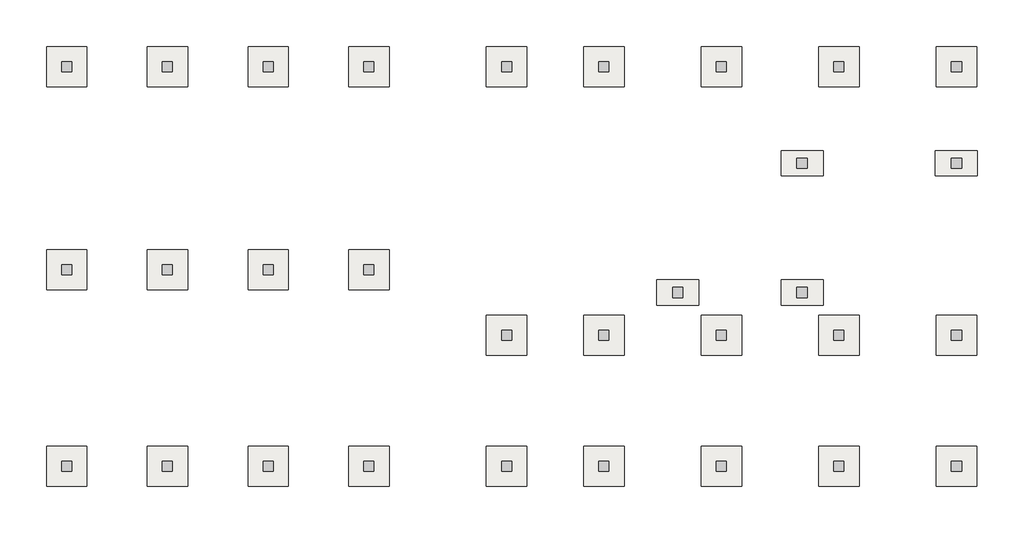
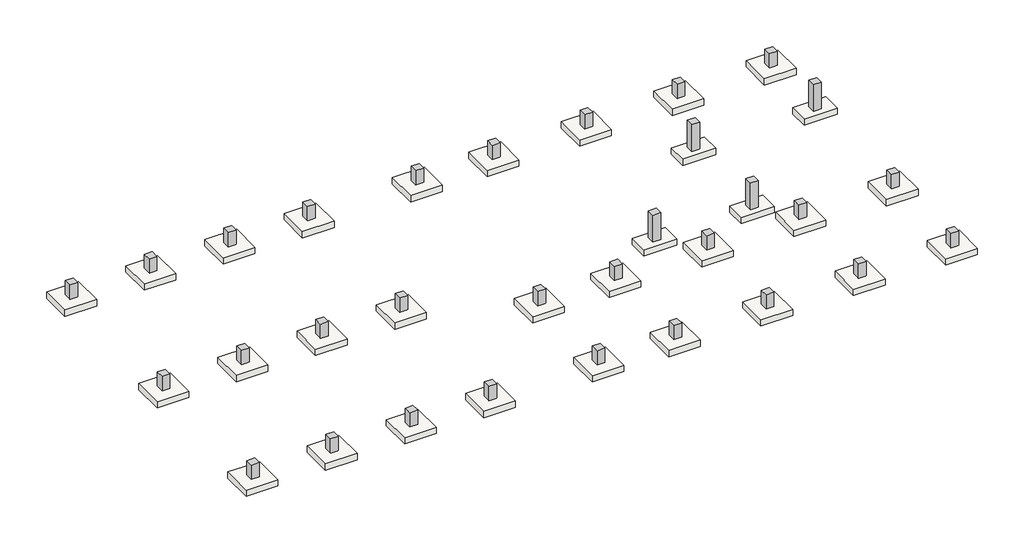
# Not in any storey: 31 columns, 31 slabs.
"""IFC4 building model written with IfcOpenShell, lengths in millimetres."""

import ifcopenshell
import ifcopenshell.guid

model = None  # the IFC model being written
_history = None  # IfcOwnerHistory: only IFC2X3 demands one
_inside = {}  # id of a spatial element -> (the spatial element, [elements in it])
_under = {}  # id of a project, library or spatial element -> (it, [spatial elements below it])
_declared = {}  # id of a project -> (the project, [libraries it declares])
_typed = {}  # id of a type object -> (the type object, [elements of that type])
_made_of = {}  # id of a material, layer set ... -> (it, [elements and type objects made of it])


def new_model(schema):
    """Start an empty IFC model of exactly this schema.

    Asked for "IFC4X3", IfcOpenShell would pick the latest addendum, in which some entities
    have other attributes; the version numbers below select the first issue.
    IFC2X3 requires an IfcOwnerHistory on every rooted entity: one is made here for all.
    """
    global model, _history
    if schema == "IFC4X3":
        model = ifcopenshell.file(schema_version=(4, 3, 0, 0))
    else:
        model = ifcopenshell.file(schema=schema)
    _inside.clear()
    _under.clear()
    _declared.clear()
    _typed.clear()
    _made_of.clear()
    _history = None
    if model.schema == "IFC2X3":
        org = make("IfcOrganization", Name="unknown")
        user = make(
            "IfcPersonAndOrganization",
            ThePerson=make("IfcPerson", FamilyName="unknown"),
            TheOrganization=org,
        )
        app = make(
            "IfcApplication",
            ApplicationDeveloper=org,
            Version="unknown",
            ApplicationFullName="unknown",
            ApplicationIdentifier="unknown",
        )
        _history = make(
            "IfcOwnerHistory",
            OwningUser=user,
            OwningApplication=app,
            ChangeAction="ADDED",
            CreationDate=0,
        )
    return model


def make(cls, **values):
    """One entity of the class cls with the attributes given. An attribute that is None is left unset."""
    return model.create_entity(
        cls, **{name: value for name, value in values.items() if value is not None}
    )


def rooted(cls, **values):
    """An entity with a GlobalId (a new one), such as an element, a storey or a relation."""
    return make(cls, GlobalId=ifcopenshell.guid.new(), OwnerHistory=_history, **values)


def si_unit(unit_type, name, prefix=None):
    """IfcSIUnit, for example si_unit("LENGTHUNIT", "METRE", prefix="MILLI")."""
    return make("IfcSIUnit", UnitType=unit_type, Prefix=prefix, Name=name)


def assignment(units):
    """IfcUnitAssignment: the units of a project."""
    return None if units is None else make("IfcUnitAssignment", Units=units)


def point(xyz):
    """IfcCartesianPoint."""
    return None if xyz is None else make("IfcCartesianPoint", Coordinates=xyz)


def direction(xyz):
    """IfcDirection."""
    return None if xyz is None else make("IfcDirection", DirectionRatios=xyz)


def frame(location, z_axis=None, x_axis=None):
    """IfcAxis2Placement3D, a coordinate frame: its origin and axes. An axis left out is left unset."""
    return make(
        "IfcAxis2Placement3D",
        Location=point(location),
        Axis=direction(z_axis),
        RefDirection=direction(x_axis),
    )


def origin():
    """The frame at (0, 0, 0) with its axes left unset."""
    return frame((0.0, 0.0, 0.0))


def place(relative_to, where):
    """IfcLocalPlacement: puts the frame where relative to a parent placement (None: the world)."""
    return make(
        "IfcLocalPlacement", PlacementRelTo=relative_to, RelativePlacement=where
    )


def context(
    kind, dimensions, precision=None, world=None, true_north=None, identifier=None
):
    """IfcGeometricRepresentationContext, for example the 3D "Model" context."""
    return make(
        "IfcGeometricRepresentationContext",
        ContextIdentifier=identifier,
        ContextType=kind,
        CoordinateSpaceDimension=dimensions,
        Precision=precision,
        WorldCoordinateSystem=world,
        TrueNorth=true_north,
    )


def project(units=None, contexts=None):
    """IfcProject with its units and contexts."""
    return rooted(
        "IfcProject",
        Name="project",
        RepresentationContexts=contexts,
        UnitsInContext=assignment(units),
    )


def spatial(cls, under=None, at=None, **own):
    """A site, building, storey or space (cls), placed at a placement, below another one or the project."""
    s = rooted(cls, ObjectPlacement=at, **own)
    if under is not None:
        _under.setdefault(under.id(), (under, []))[1].append(s)
    return s


def polyline(points):
    """IfcPolyline through the points."""
    return make("IfcPolyline", Points=[point(p) for p in points])


def outline(outer, holes=None, kind="AREA"):
    """IfcArbitraryClosedProfileDef: a profile drawn as a closed curve; with holes, ...WithVoids."""
    if holes is None:
        return make("IfcArbitraryClosedProfileDef", ProfileType=kind, OuterCurve=outer)
    return make(
        "IfcArbitraryProfileDefWithVoids",
        ProfileType=kind,
        OuterCurve=outer,
        InnerCurves=holes,
    )


def extrude(swept, where, along, depth):
    """IfcExtrudedAreaSolid: the profile swept, set in the frame where, extruded along a direction by depth."""
    return make(
        "IfcExtrudedAreaSolid",
        SweptArea=swept,
        Position=where,
        ExtrudedDirection=direction(along),
        Depth=depth,
    )


def shape(context_of_items, identifier, shape_type, items):
    """IfcShapeRepresentation: the items that make up one representation, for example the "Body"."""
    return make(
        "IfcShapeRepresentation",
        ContextOfItems=context_of_items,
        RepresentationIdentifier=identifier,
        RepresentationType=shape_type,
        Items=items,
    )


def source(mapping_origin, context_of_items, identifier, shape_type, items):
    """IfcRepresentationMap: a shape defined once, which mapped items show again and again."""
    return make(
        "IfcRepresentationMap",
        MappingOrigin=mapping_origin,
        MappedRepresentation=shape(context_of_items, identifier, shape_type, items),
    )


def transform(
    local_origin,
    x_axis=None,
    y_axis=None,
    z_axis=None,
    scale=None,
    scale2=None,
    scale3=None,
    uniform=True,
):
    """IfcCartesianTransformationOperator3D, or its non-uniform kind. x_axis, y_axis, z_axis: its Axis1, 2, 3."""
    if uniform:
        return make(
            "IfcCartesianTransformationOperator3D",
            Axis1=direction(x_axis),
            Axis2=direction(y_axis),
            LocalOrigin=point(local_origin),
            Scale=scale,
            Axis3=direction(z_axis),
        )
    return make(
        "IfcCartesianTransformationOperator3DnonUniform",
        Axis1=direction(x_axis),
        Axis2=direction(y_axis),
        LocalOrigin=point(local_origin),
        Scale=scale,
        Axis3=direction(z_axis),
        Scale2=scale2,
        Scale3=scale3,
    )


def mapped(mapping_source, mapping_target):
    """IfcMappedItem: shows the shape of a source again, moved by a transform."""
    return make(
        "IfcMappedItem", MappingSource=mapping_source, MappingTarget=mapping_target
    )


def made_of(thing, what):
    """Note that an element or type object is made of a material, layer set ...; save() writes the relation."""
    if what is not None:
        _made_of.setdefault(what.id(), (what, []))[1].append(thing)
    return thing


def element(
    cls,
    number,
    at=None,
    inside=None,
    cuts=None,
    type_object=None,
    material=None,
    context=None,
    identifier="Body",
    shape_type=None,
    held_by="IfcProductDefinitionShape",
    body=None,
    shapes=None,
    **own,
):
    """One element of the class cls, such as IfcWall. Its Tag is "e" and its number.

    at: its placement. inside: the storey or other place that contains it. cuts: it is an
    opening in that element (IfcRelVoidsElement). A single representation is given by context,
    identifier, shape_type and body (its items); several are given by shapes. held_by: the class
    of the entity that holds the representations. save() writes the other relations.
    """
    e = rooted(cls, Tag="e%d" % number, ObjectPlacement=at, **own)
    if body is not None:
        shapes = [shape(context, identifier, shape_type, body)]
    if shapes is not None:
        e.Representation = make(held_by, Representations=shapes)
    if inside is not None:
        _inside.setdefault(inside.id(), (inside, []))[1].append(e)
    if cuts is not None:
        rooted(
            "IfcRelVoidsElement", RelatingBuildingElement=cuts, RelatedOpeningElement=e
        )
    if type_object is not None:
        _typed.setdefault(type_object.id(), (type_object, []))[1].append(e)
    return made_of(e, material)


def aggregate(whole, parts):
    """IfcRelAggregates: a whole, such as a stair, and the parts it consists of."""
    return rooted("IfcRelAggregates", RelatingObject=whole, RelatedObjects=parts)


def save(model, path):
    """Write the relations noted so far, then the file.

    IfcRelAggregates (storeys below a building ...), IfcRelContainedInSpatialStructure (elements
    in a storey), IfcRelDefinesByType, IfcRelAssociatesMaterial and IfcRelDeclares: one each for
    every whole, place, type object, material and project.
    """
    for whole, parts in _under.values():
        aggregate(whole, parts)
    for where, things in _inside.values():
        rooted(
            "IfcRelContainedInSpatialStructure",
            RelatedElements=things,
            RelatingStructure=where,
        )
    for kind, things in _typed.values():
        rooted("IfcRelDefinesByType", RelatedObjects=things, RelatingType=kind)
    for what, things in _made_of.values():
        rooted("IfcRelAssociatesMaterial", RelatedObjects=things, RelatingMaterial=what)
    for by, libraries in _declared.values():
        rooted("IfcRelDeclares", RelatingContext=by, RelatedDefinitions=libraries)
    model.write(path)


def ft211_footing_rectangular_r1_5fe39465(model_context):
    return source(origin(), model_context, "Body", "SweptSolid", [
        extrude(outline(polyline([(1200.0, 1200.0), (1200.0, -1200.0), (-1200.0, -1200.0), (-1200.0, 1200.0), (1200.0, 1200.0)])), frame((0.0, 0.0, -500.0), z_axis=(0.0, 0.0, 1.0), x_axis=(1.0, 0.0, 0.0)), (0.0, 0.0, 1.0), 500.0),
    ])


def ft211_footing_rectangular_r1_907a7f09(model_context):
    return source(origin(), model_context, "Body", "SweptSolid", [
        extrude(outline(polyline([(1250.0, 750.0), (1250.0, -750.0), (-1250.0, -750.0), (-1250.0, 750.0), (1250.0, 750.0)])), frame((0.0, 0.0, -500.0), z_axis=(0.0, 0.0, 1.0), x_axis=(1.0, 0.0, 0.0)), (0.0, 0.0, 1.0), 500.0),
    ])


model = new_model("IFC4")

# Units and contexts
model_context = context("Model", 3, world=origin())
ifc_project = project(units=[si_unit("LENGTHUNIT", "METRE", prefix="MILLI")], contexts=[model_context])

# Site, building
site = spatial("IfcSite", under=ifc_project)
building = spatial("IfcBuilding", under=site)

# Columns
placement = place(None, origin())
element("IfcColumn", 1, ObjectType="RC_Column_Rectangular : H_SC_ACC_UG PED_W600xL600", at=placement, inside=building, context=model_context, shape_type="SweptSolid", body=[
    extrude(outline(polyline([(224.7, 12616.5208589), (224.7, 12016.5208589), (-375.3, 12016.5208589), (-375.3, 12616.5208589), (224.7, 12616.5208589)])), frame((0.0, 0.0, -1000.0), z_axis=(0.0, 0.0, 1.0), x_axis=(1.0, 0.0, 0.0)), (0.0, 0.0, 1.0), 1150.0),
])
element("IfcColumn", 2, ObjectType="RC_Column_Rectangular : H_SC_ACC_UG PED_W600xL600", at=placement, inside=building, context=model_context, shape_type="SweptSolid", body=[
    extrude(outline(polyline([(6224.7, 12616.5208589), (6224.7, 12016.5208589), (5624.7, 12016.5208589), (5624.7, 12616.5208589), (6224.7, 12616.5208589)])), frame((0.0, 0.0, -1000.0), z_axis=(0.0, 0.0, 1.0), x_axis=(1.0, 0.0, 0.0)), (0.0, 0.0, 1.0), 1150.0),
])
element("IfcColumn", 3, ObjectType="RC_Column_Rectangular : H_SC_ACC_UG PED_W600xL600", at=placement, inside=building, context=model_context, shape_type="SweptSolid", body=[
    extrude(outline(polyline([(12224.7, 12616.5208589), (12224.7, 12016.5208589), (11624.7, 12016.5208589), (11624.7, 12616.5208589), (12224.7, 12616.5208589)])), frame((0.0, 0.0, -1000.0), z_axis=(0.0, 0.0, 1.0), x_axis=(1.0, 0.0, 0.0)), (0.0, 0.0, 1.0), 1150.0),
])
element("IfcColumn", 4, ObjectType="RC_Column_Rectangular : H_SC_ACC_UG PED_W600xL600", at=placement, inside=building, context=model_context, shape_type="SweptSolid", body=[
    extrude(outline(polyline([(18224.7, 12616.5208589), (18224.7, 12016.5208589), (17624.7, 12016.5208589), (17624.7, 12616.5208589), (18224.7, 12616.5208589)])), frame((0.0, 0.0, -1000.0), z_axis=(0.0, 0.0, 1.0), x_axis=(1.0, 0.0, 0.0)), (0.0, 0.0, 1.0), 1150.0),
])
element("IfcColumn", 5, ObjectType="RC_Column_Rectangular : H_SC_ACC_UG PED_W600xL600", at=placement, inside=building, context=model_context, shape_type="SweptSolid", body=[
    extrude(outline(polyline([(224.7, 24716.5208589), (224.7, 24116.5208589), (-375.3, 24116.5208589), (-375.3, 24716.5208589), (224.7, 24716.5208589)])), frame((0.0, 0.0, -1000.0), z_axis=(0.0, 0.0, 1.0), x_axis=(1.0, 0.0, 0.0)), (0.0, 0.0, 1.0), 1150.0),
])
element("IfcColumn", 6, ObjectType="RC_Column_Rectangular : H_SC_ACC_UG PED_W600xL600", at=placement, inside=building, context=model_context, shape_type="SweptSolid", body=[
    extrude(outline(polyline([(6224.7, 24716.5208589), (6224.7, 24116.5208589), (5624.7, 24116.5208589), (5624.7, 24716.5208589), (6224.7, 24716.5208589)])), frame((0.0, 0.0, -1000.0), z_axis=(0.0, 0.0, 1.0), x_axis=(1.0, 0.0, 0.0)), (0.0, 0.0, 1.0), 1150.0),
])
element("IfcColumn", 7, ObjectType="RC_Column_Rectangular : H_SC_ACC_UG PED_W600xL600", at=placement, inside=building, context=model_context, shape_type="SweptSolid", body=[
    extrude(outline(polyline([(12224.7, 24716.5208589), (12224.7, 24116.5208589), (11624.7, 24116.5208589), (11624.7, 24716.5208589), (12224.7, 24716.5208589)])), frame((0.0, 0.0, -1000.0), z_axis=(0.0, 0.0, 1.0), x_axis=(1.0, 0.0, 0.0)), (0.0, 0.0, 1.0), 1150.0),
])
element("IfcColumn", 8, ObjectType="RC_Column_Rectangular : H_SC_ACC_UG PED_W600xL600", at=placement, inside=building, context=model_context, shape_type="SweptSolid", body=[
    extrude(outline(polyline([(18224.7, 24716.5208589), (18224.7, 24116.5208589), (17624.7, 24116.5208589), (17624.7, 24716.5208589), (18224.7, 24716.5208589)])), frame((0.0, 0.0, -1000.0), z_axis=(0.0, 0.0, 1.0), x_axis=(1.0, 0.0, 0.0)), (0.0, 0.0, 1.0), 1150.0),
])
element("IfcColumn", 9, ObjectType="RC_Column_Rectangular : H_SC_ACC_UG PED_W600xL600", at=placement, inside=building, context=model_context, shape_type="SweptSolid", body=[
    extrude(outline(polyline([(26424.7, 24716.5208589), (26424.7, 24116.5208589), (25824.7, 24116.5208589), (25824.7, 24716.5208589), (26424.7, 24716.5208589)])), frame((0.0, 0.0, -1000.0), z_axis=(0.0, 0.0, 1.0), x_axis=(1.0, 0.0, 0.0)), (0.0, 0.0, 1.0), 1150.0),
])
element("IfcColumn", 10, ObjectType="RC_Column_Rectangular : H_SC_ACC_UG PED_W600xL600", at=placement, inside=building, context=model_context, shape_type="SweptSolid", body=[
    extrude(outline(polyline([(32224.7, 24716.5208589), (32224.7, 24116.5208589), (31624.7, 24116.5208589), (31624.7, 24716.5208589), (32224.7, 24716.5208589)])), frame((0.0, 0.0, -1000.0), z_axis=(0.0, 0.0, 1.0), x_axis=(1.0, 0.0, 0.0)), (0.0, 0.0, 1.0), 1150.0),
])
element("IfcColumn", 11, ObjectType="RC_Column_Rectangular : H_SC_ACC_UG PED_W600xL600", at=placement, inside=building, context=model_context, shape_type="SweptSolid", body=[
    extrude(outline(polyline([(39224.7, 24716.5208589), (39224.7, 24116.5208589), (38624.7, 24116.5208589), (38624.7, 24716.5208589), (39224.7, 24716.5208589)])), frame((0.0, 0.0, -1000.0), z_axis=(0.0, 0.0, 1.0), x_axis=(1.0, 0.0, 0.0)), (0.0, 0.0, 1.0), 1150.0),
])
element("IfcColumn", 12, ObjectType="RC_Column_Rectangular : H_SC_ACC_UG PED_W600xL600", at=placement, inside=building, context=model_context, shape_type="SweptSolid", body=[
    extrude(outline(polyline([(46224.7, 24716.5208589), (46224.7, 24116.5208589), (45624.7, 24116.5208589), (45624.7, 24716.5208589), (46224.7, 24716.5208589)])), frame((0.0, 0.0, -1000.0), z_axis=(0.0, 0.0, 1.0), x_axis=(1.0, 0.0, 0.0)), (0.0, 0.0, 1.0), 1150.0),
])
element("IfcColumn", 13, ObjectType="RC_Column_Rectangular : H_SC_ACC_UG PED_W600xL600", at=placement, inside=building, context=model_context, shape_type="SweptSolid", body=[
    extrude(outline(polyline([(53224.7, 24716.5208589), (53224.7, 24116.5208589), (52624.7, 24116.5208589), (52624.7, 24716.5208589), (53224.7, 24716.5208589)])), frame((0.0, 0.0, -1000.0), z_axis=(0.0, 0.0, 1.0), x_axis=(1.0, 0.0, 0.0)), (0.0, 0.0, 1.0), 1150.0),
])
element("IfcColumn", 14, ObjectType="RC_Column_Rectangular : H_SC_ACC_UG PED_W600xL600", at=placement, inside=building, context=model_context, shape_type="SweptSolid", body=[
    extrude(outline(polyline([(26424.7, 8716.5208589), (26424.7, 8116.5208589), (25824.7, 8116.5208589), (25824.7, 8716.5208589), (26424.7, 8716.5208589)])), frame((0.0, 0.0, -1000.0), z_axis=(0.0, 0.0, 1.0), x_axis=(1.0, 0.0, 0.0)), (0.0, 0.0, 1.0), 1150.0),
])
element("IfcColumn", 15, ObjectType="RC_Column_Rectangular : H_SC_ACC_UG PED_W600xL600", at=placement, inside=building, context=model_context, shape_type="SweptSolid", body=[
    extrude(outline(polyline([(32224.7, 8716.5208589), (32224.7, 8116.5208589), (31624.7, 8116.5208589), (31624.7, 8716.5208589), (32224.7, 8716.5208589)])), frame((0.0, 0.0, -1000.0), z_axis=(0.0, 0.0, 1.0), x_axis=(1.0, 0.0, 0.0)), (0.0, 0.0, 1.0), 1150.0),
])
element("IfcColumn", 16, ObjectType="RC_Column_Rectangular : H_SC_ACC_UG PED_W600xL600", at=placement, inside=building, context=model_context, shape_type="SweptSolid", body=[
    extrude(outline(polyline([(39224.7, 8716.5208589), (39224.7, 8116.5208589), (38624.7, 8116.5208589), (38624.7, 8716.5208589), (39224.7, 8716.5208589)])), frame((0.0, 0.0, -1000.0), z_axis=(0.0, 0.0, 1.0), x_axis=(1.0, 0.0, 0.0)), (0.0, 0.0, 1.0), 1150.0),
])
element("IfcColumn", 17, ObjectType="RC_Column_Rectangular : H_SC_ACC_UG PED_W600xL600", at=placement, inside=building, context=model_context, shape_type="SweptSolid", body=[
    extrude(outline(polyline([(46224.7, 8716.5208589), (46224.7, 8116.5208589), (45624.7, 8116.5208589), (45624.7, 8716.5208589), (46224.7, 8716.5208589)])), frame((0.0, 0.0, -1000.0), z_axis=(0.0, 0.0, 1.0), x_axis=(1.0, 0.0, 0.0)), (0.0, 0.0, 1.0), 1150.0),
])
element("IfcColumn", 18, ObjectType="RC_Column_Rectangular : H_SC_ACC_UG PED_W600xL600", at=placement, inside=building, context=model_context, shape_type="SweptSolid", body=[
    extrude(outline(polyline([(53224.7, 8716.5208589), (53224.7, 8116.5208589), (52624.7, 8116.5208589), (52624.7, 8716.5208589), (53224.7, 8716.5208589)])), frame((0.0, 0.0, -1000.0), z_axis=(0.0, 0.0, 1.0), x_axis=(1.0, 0.0, 0.0)), (0.0, 0.0, 1.0), 1150.0),
])
element("IfcColumn", 19, ObjectType="RC_Column_Rectangular : H_SC_ACC_UG PED_W600xL600", at=placement, inside=building, context=model_context, shape_type="SweptSolid", body=[
    extrude(outline(polyline([(224.7, 916.5208589), (224.7, 316.5208589), (-375.3, 316.5208589), (-375.3, 916.5208589), (224.7, 916.5208589)])), frame((0.0, 0.0, -1000.0), z_axis=(0.0, 0.0, 1.0), x_axis=(1.0, 0.0, 0.0)), (0.0, 0.0, 1.0), 1150.0),
])
element("IfcColumn", 20, ObjectType="RC_Column_Rectangular : H_SC_ACC_UG PED_W600xL600", at=placement, inside=building, context=model_context, shape_type="SweptSolid", body=[
    extrude(outline(polyline([(6224.7, 916.5208589), (6224.7, 316.5208589), (5624.7, 316.5208589), (5624.7, 916.5208589), (6224.7, 916.5208589)])), frame((0.0, 0.0, -1000.0), z_axis=(0.0, 0.0, 1.0), x_axis=(1.0, 0.0, 0.0)), (0.0, 0.0, 1.0), 1150.0),
])
element("IfcColumn", 21, ObjectType="RC_Column_Rectangular : H_SC_ACC_UG PED_W600xL600", at=placement, inside=building, context=model_context, shape_type="SweptSolid", body=[
    extrude(outline(polyline([(12224.7, 916.5208589), (12224.7, 316.5208589), (11624.7, 316.5208589), (11624.7, 916.5208589), (12224.7, 916.5208589)])), frame((0.0, 0.0, -1000.0), z_axis=(0.0, 0.0, 1.0), x_axis=(1.0, 0.0, 0.0)), (0.0, 0.0, 1.0), 1150.0),
])
element("IfcColumn", 22, ObjectType="RC_Column_Rectangular : H_SC_ACC_UG PED_W600xL600", at=placement, inside=building, context=model_context, shape_type="SweptSolid", body=[
    extrude(outline(polyline([(18224.7, 916.5208589), (18224.7, 316.5208589), (17624.7, 316.5208589), (17624.7, 916.5208589), (18224.7, 916.5208589)])), frame((0.0, 0.0, -1000.0), z_axis=(0.0, 0.0, 1.0), x_axis=(1.0, 0.0, 0.0)), (0.0, 0.0, 1.0), 1150.0),
])
element("IfcColumn", 23, ObjectType="RC_Column_Rectangular : H_SC_ACC_UG PED_W600xL600", at=placement, inside=building, context=model_context, shape_type="SweptSolid", body=[
    extrude(outline(polyline([(26424.7, 916.5208589), (26424.7, 316.5208589), (25824.7, 316.5208589), (25824.7, 916.5208589), (26424.7, 916.5208589)])), frame((0.0, 0.0, -1000.0), z_axis=(0.0, 0.0, 1.0), x_axis=(1.0, 0.0, 0.0)), (0.0, 0.0, 1.0), 1150.0),
])
element("IfcColumn", 24, ObjectType="RC_Column_Rectangular : H_SC_ACC_UG PED_W600xL600", at=placement, inside=building, context=model_context, shape_type="SweptSolid", body=[
    extrude(outline(polyline([(32224.7, 916.5208589), (32224.7, 316.5208589), (31624.7, 316.5208589), (31624.7, 916.5208589), (32224.7, 916.5208589)])), frame((0.0, 0.0, -1000.0), z_axis=(0.0, 0.0, 1.0), x_axis=(1.0, 0.0, 0.0)), (0.0, 0.0, 1.0), 1150.0),
])
element("IfcColumn", 25, ObjectType="RC_Column_Rectangular : H_SC_ACC_UG PED_W600xL600", at=placement, inside=building, context=model_context, shape_type="SweptSolid", body=[
    extrude(outline(polyline([(39224.7, 916.5208589), (39224.7, 316.5208589), (38624.7, 316.5208589), (38624.7, 916.5208589), (39224.7, 916.5208589)])), frame((0.0, 0.0, -1000.0), z_axis=(0.0, 0.0, 1.0), x_axis=(1.0, 0.0, 0.0)), (0.0, 0.0, 1.0), 1150.0),
])
element("IfcColumn", 26, ObjectType="RC_Column_Rectangular : H_SC_ACC_UG PED_W600xL600", at=placement, inside=building, context=model_context, shape_type="SweptSolid", body=[
    extrude(outline(polyline([(46224.7, 916.5208589), (46224.7, 316.5208589), (45624.7, 316.5208589), (45624.7, 916.5208589), (46224.7, 916.5208589)])), frame((0.0, 0.0, -1000.0), z_axis=(0.0, 0.0, 1.0), x_axis=(1.0, 0.0, 0.0)), (0.0, 0.0, 1.0), 1150.0),
])
element("IfcColumn", 27, ObjectType="RC_Column_Rectangular : H_SC_ACC_UG PED_W600xL600", at=placement, inside=building, context=model_context, shape_type="SweptSolid", body=[
    extrude(outline(polyline([(53224.7, 916.5208589), (53224.7, 316.5208589), (52624.7, 316.5208589), (52624.7, 916.5208589), (53224.7, 916.5208589)])), frame((0.0, 0.0, -1000.0), z_axis=(0.0, 0.0, 1.0), x_axis=(1.0, 0.0, 0.0)), (0.0, 0.0, 1.0), 1150.0),
])
element("IfcColumn", 28, ObjectType="RC_Column_Rectangular : H_SC_ACC_UG PED_W600xL600", at=placement, inside=building, context=model_context, shape_type="SweptSolid", body=[
    extrude(outline(polyline([(36624.7, 11266.5208589), (36624.7, 10666.5208589), (36024.7, 10666.5208589), (36024.7, 11266.5208589), (36624.7, 11266.5208589)])), frame((0.0, 0.0, -1000.0), z_axis=(0.0, 0.0, 1.0), x_axis=(1.0, 0.0, 0.0)), (0.0, 0.0, 1.0), 2150.0),
])
element("IfcColumn", 29, ObjectType="RC_Column_Rectangular : H_SC_ACC_UG PED_W600xL600", at=placement, inside=building, context=model_context, shape_type="SweptSolid", body=[
    extrude(outline(polyline([(44024.7, 11266.5208589), (44024.7, 10666.5208589), (43424.7, 10666.5208589), (43424.7, 11266.5208589), (44024.7, 11266.5208589)])), frame((0.0, 0.0, -1000.0), z_axis=(0.0, 0.0, 1.0), x_axis=(1.0, 0.0, 0.0)), (0.0, 0.0, 1.0), 2150.0),
])
element("IfcColumn", 30, ObjectType="RC_Column_Rectangular : H_SC_ACC_UG PED_W600xL600", at=placement, inside=building, context=model_context, shape_type="SweptSolid", body=[
    extrude(outline(polyline([(44024.7, 18966.5208589), (44024.7, 18366.5208589), (43424.7, 18366.5208589), (43424.7, 18966.5208589), (44024.7, 18966.5208589)])), frame((0.0, 0.0, -1000.0), z_axis=(0.0, 0.0, 1.0), x_axis=(1.0, 0.0, 0.0)), (0.0, 0.0, 1.0), 2150.0),
])
element("IfcColumn", 31, ObjectType="RC_Column_Rectangular : H_SC_ACC_UG PED_W600xL600", at=placement, inside=building, context=model_context, shape_type="SweptSolid", body=[
    extrude(outline(polyline([(53224.7, 18966.5208589), (53224.7, 18366.5208589), (52624.7, 18366.5208589), (52624.7, 18966.5208589), (53224.7, 18966.5208589)])), frame((0.0, 0.0, -1000.0), z_axis=(0.0, 0.0, 1.0), x_axis=(1.0, 0.0, 0.0)), (0.0, 0.0, 1.0), 2150.0),
])

# Slabs
ft211_footing_rectangular_r1_shape = ft211_footing_rectangular_r1_5fe39465(model_context)
element("IfcSlab", 32, ObjectType="FT211-Footing-Rectangular_R1 : H_SF_ACF_W2400xL2400xT500_Bitumen", at=placement, inside=building, context=model_context, shape_type="MappedRepresentation", body=[
    mapped(ft211_footing_rectangular_r1_shape, transform((-75.3, 12316.5208589, -1000.0), x_axis=(1.0, 0.0, 0.0), y_axis=(0.0, 1.0, 0.0), z_axis=(0.0, 0.0, 1.0))),
])
element("IfcSlab", 33, ObjectType="FT211-Footing-Rectangular_R1 : H_SF_ACF_W2400xL2400xT500_Bitumen", at=placement, inside=building, context=model_context, shape_type="MappedRepresentation", body=[
    mapped(ft211_footing_rectangular_r1_shape, transform((5924.7, 12316.5208589, -1000.0), x_axis=(1.0, 0.0, 0.0), y_axis=(0.0, 1.0, 0.0), z_axis=(0.0, 0.0, 1.0))),
])
element("IfcSlab", 34, ObjectType="FT211-Footing-Rectangular_R1 : H_SF_ACF_W2400xL2400xT500_Bitumen", at=placement, inside=building, context=model_context, shape_type="MappedRepresentation", body=[
    mapped(ft211_footing_rectangular_r1_shape, transform((11924.7, 12316.5208589, -1000.0), x_axis=(1.0, 0.0, 0.0), y_axis=(0.0, 1.0, 0.0), z_axis=(0.0, 0.0, 1.0))),
])
element("IfcSlab", 35, ObjectType="FT211-Footing-Rectangular_R1 : H_SF_ACF_W2400xL2400xT500_Bitumen", at=placement, inside=building, context=model_context, shape_type="MappedRepresentation", body=[
    mapped(ft211_footing_rectangular_r1_shape, transform((17924.7, 12316.5208589, -1000.0), x_axis=(1.0, 0.0, 0.0), y_axis=(0.0, 1.0, 0.0), z_axis=(0.0, 0.0, 1.0))),
])
element("IfcSlab", 36, ObjectType="FT211-Footing-Rectangular_R1 : H_SF_ACF_W2400xL2400xT500_Bitumen", at=placement, inside=building, context=model_context, shape_type="MappedRepresentation", body=[
    mapped(ft211_footing_rectangular_r1_shape, transform((-75.3, 24416.5208589, -1000.0), x_axis=(1.0, 0.0, 0.0), y_axis=(0.0, 1.0, 0.0), z_axis=(0.0, 0.0, 1.0))),
])
element("IfcSlab", 37, ObjectType="FT211-Footing-Rectangular_R1 : H_SF_ACF_W2400xL2400xT500_Bitumen", at=placement, inside=building, context=model_context, shape_type="MappedRepresentation", body=[
    mapped(ft211_footing_rectangular_r1_shape, transform((5924.7, 24416.5208589, -1000.0), x_axis=(1.0, 0.0, 0.0), y_axis=(0.0, 1.0, 0.0), z_axis=(0.0, 0.0, 1.0))),
])
element("IfcSlab", 38, ObjectType="FT211-Footing-Rectangular_R1 : H_SF_ACF_W2400xL2400xT500_Bitumen", at=placement, inside=building, context=model_context, shape_type="MappedRepresentation", body=[
    mapped(ft211_footing_rectangular_r1_shape, transform((11924.7, 24416.5208589, -1000.0), x_axis=(1.0, 0.0, 0.0), y_axis=(0.0, 1.0, 0.0), z_axis=(0.0, 0.0, 1.0))),
])
element("IfcSlab", 39, ObjectType="FT211-Footing-Rectangular_R1 : H_SF_ACF_W2400xL2400xT500_Bitumen", at=placement, inside=building, context=model_context, shape_type="MappedRepresentation", body=[
    mapped(ft211_footing_rectangular_r1_shape, transform((17924.7, 24416.5208589, -1000.0), x_axis=(1.0, 0.0, 0.0), y_axis=(0.0, 1.0, 0.0), z_axis=(0.0, 0.0, 1.0))),
])
element("IfcSlab", 40, ObjectType="FT211-Footing-Rectangular_R1 : H_SF_ACF_W2400xL2400xT500_Bitumen", at=placement, inside=building, context=model_context, shape_type="MappedRepresentation", body=[
    mapped(ft211_footing_rectangular_r1_shape, transform((26124.7, 24416.5208589, -1000.0), x_axis=(1.0, 0.0, 0.0), y_axis=(0.0, 1.0, 0.0), z_axis=(0.0, 0.0, 1.0))),
])
element("IfcSlab", 41, ObjectType="FT211-Footing-Rectangular_R1 : H_SF_ACF_W2400xL2400xT500_Bitumen", at=placement, inside=building, context=model_context, shape_type="MappedRepresentation", body=[
    mapped(ft211_footing_rectangular_r1_shape, transform((31924.7, 24416.5208589, -1000.0), x_axis=(1.0, 0.0, 0.0), y_axis=(0.0, 1.0, 0.0), z_axis=(0.0, 0.0, 1.0))),
])
element("IfcSlab", 42, ObjectType="FT211-Footing-Rectangular_R1 : H_SF_ACF_W2400xL2400xT500_Bitumen", at=placement, inside=building, context=model_context, shape_type="MappedRepresentation", body=[
    mapped(ft211_footing_rectangular_r1_shape, transform((38924.7, 24416.5208589, -1000.0), x_axis=(1.0, 0.0, 0.0), y_axis=(0.0, 1.0, 0.0), z_axis=(0.0, 0.0, 1.0))),
])
element("IfcSlab", 43, ObjectType="FT211-Footing-Rectangular_R1 : H_SF_ACF_W2400xL2400xT500_Bitumen", at=placement, inside=building, context=model_context, shape_type="MappedRepresentation", body=[
    mapped(ft211_footing_rectangular_r1_shape, transform((45924.7, 24416.5208589, -1000.0), x_axis=(1.0, 0.0, 0.0), y_axis=(0.0, 1.0, 0.0), z_axis=(0.0, 0.0, 1.0))),
])
element("IfcSlab", 44, ObjectType="FT211-Footing-Rectangular_R1 : H_SF_ACF_W2400xL2400xT500_Bitumen", at=placement, inside=building, context=model_context, shape_type="MappedRepresentation", body=[
    mapped(ft211_footing_rectangular_r1_shape, transform((52924.7, 24416.5208589, -1000.0), x_axis=(1.0, 0.0, 0.0), y_axis=(0.0, 1.0, 0.0), z_axis=(0.0, 0.0, 1.0))),
])
element("IfcSlab", 45, ObjectType="FT211-Footing-Rectangular_R1 : H_SF_ACF_W2400xL2400xT500_Bitumen", at=placement, inside=building, context=model_context, shape_type="MappedRepresentation", body=[
    mapped(ft211_footing_rectangular_r1_shape, transform((26124.7, 8416.5208589, -1000.0), x_axis=(1.0, 0.0, 0.0), y_axis=(0.0, 1.0, 0.0), z_axis=(0.0, 0.0, 1.0))),
])
element("IfcSlab", 46, ObjectType="FT211-Footing-Rectangular_R1 : H_SF_ACF_W2400xL2400xT500_Bitumen", at=placement, inside=building, context=model_context, shape_type="MappedRepresentation", body=[
    mapped(ft211_footing_rectangular_r1_shape, transform((31924.7, 8416.5208589, -1000.0), x_axis=(1.0, 0.0, 0.0), y_axis=(0.0, 1.0, 0.0), z_axis=(0.0, 0.0, 1.0))),
])
element("IfcSlab", 47, ObjectType="FT211-Footing-Rectangular_R1 : H_SF_ACF_W2400xL2400xT500_Bitumen", at=placement, inside=building, context=model_context, shape_type="MappedRepresentation", body=[
    mapped(ft211_footing_rectangular_r1_shape, transform((38924.7, 8416.5208589, -1000.0), x_axis=(1.0, 0.0, 0.0), y_axis=(0.0, 1.0, 0.0), z_axis=(0.0, 0.0, 1.0))),
])
element("IfcSlab", 48, ObjectType="FT211-Footing-Rectangular_R1 : H_SF_ACF_W2400xL2400xT500_Bitumen", at=placement, inside=building, context=model_context, shape_type="MappedRepresentation", body=[
    mapped(ft211_footing_rectangular_r1_shape, transform((45924.7, 8416.5208589, -1000.0), x_axis=(1.0, 0.0, 0.0), y_axis=(0.0, 1.0, 0.0), z_axis=(0.0, 0.0, 1.0))),
])
element("IfcSlab", 49, ObjectType="FT211-Footing-Rectangular_R1 : H_SF_ACF_W2400xL2400xT500_Bitumen", at=placement, inside=building, context=model_context, shape_type="MappedRepresentation", body=[
    mapped(ft211_footing_rectangular_r1_shape, transform((52924.7, 8416.5208589, -1000.0), x_axis=(1.0, 0.0, 0.0), y_axis=(0.0, 1.0, 0.0), z_axis=(0.0, 0.0, 1.0))),
])
element("IfcSlab", 50, ObjectType="FT211-Footing-Rectangular_R1 : H_SF_ACF_W2400xL2400xT500_Bitumen", at=placement, inside=building, context=model_context, shape_type="MappedRepresentation", body=[
    mapped(ft211_footing_rectangular_r1_shape, transform((-75.3, 616.5208589, -1000.0), x_axis=(1.0, 0.0, 0.0), y_axis=(0.0, 1.0, 0.0), z_axis=(0.0, 0.0, 1.0))),
])
element("IfcSlab", 51, ObjectType="FT211-Footing-Rectangular_R1 : H_SF_ACF_W2400xL2400xT500_Bitumen", at=placement, inside=building, context=model_context, shape_type="MappedRepresentation", body=[
    mapped(ft211_footing_rectangular_r1_shape, transform((5924.7, 616.5208589, -1000.0), x_axis=(1.0, 0.0, 0.0), y_axis=(0.0, 1.0, 0.0), z_axis=(0.0, 0.0, 1.0))),
])
element("IfcSlab", 52, ObjectType="FT211-Footing-Rectangular_R1 : H_SF_ACF_W2400xL2400xT500_Bitumen", at=placement, inside=building, context=model_context, shape_type="MappedRepresentation", body=[
    mapped(ft211_footing_rectangular_r1_shape, transform((11924.7, 616.5208589, -1000.0), x_axis=(1.0, 0.0, 0.0), y_axis=(0.0, 1.0, 0.0), z_axis=(0.0, 0.0, 1.0))),
])
element("IfcSlab", 53, ObjectType="FT211-Footing-Rectangular_R1 : H_SF_ACF_W2400xL2400xT500_Bitumen", at=placement, inside=building, context=model_context, shape_type="MappedRepresentation", body=[
    mapped(ft211_footing_rectangular_r1_shape, transform((17924.7, 616.5208589, -1000.0), x_axis=(1.0, 0.0, 0.0), y_axis=(0.0, 1.0, 0.0), z_axis=(0.0, 0.0, 1.0))),
])
element("IfcSlab", 54, ObjectType="FT211-Footing-Rectangular_R1 : H_SF_ACF_W2400xL2400xT500_Bitumen", at=placement, inside=building, context=model_context, shape_type="MappedRepresentation", body=[
    mapped(ft211_footing_rectangular_r1_shape, transform((26124.7, 616.5208589, -1000.0), x_axis=(1.0, 0.0, 0.0), y_axis=(0.0, 1.0, 0.0), z_axis=(0.0, 0.0, 1.0))),
])
element("IfcSlab", 55, ObjectType="FT211-Footing-Rectangular_R1 : H_SF_ACF_W2400xL2400xT500_Bitumen", at=placement, inside=building, context=model_context, shape_type="MappedRepresentation", body=[
    mapped(ft211_footing_rectangular_r1_shape, transform((31924.7, 616.5208589, -1000.0), x_axis=(1.0, 0.0, 0.0), y_axis=(0.0, 1.0, 0.0), z_axis=(0.0, 0.0, 1.0))),
])
element("IfcSlab", 56, ObjectType="FT211-Footing-Rectangular_R1 : H_SF_ACF_W2400xL2400xT500_Bitumen", at=placement, inside=building, context=model_context, shape_type="MappedRepresentation", body=[
    mapped(ft211_footing_rectangular_r1_shape, transform((38924.7, 616.5208589, -1000.0), x_axis=(1.0, 0.0, 0.0), y_axis=(0.0, 1.0, 0.0), z_axis=(0.0, 0.0, 1.0))),
])
element("IfcSlab", 57, ObjectType="FT211-Footing-Rectangular_R1 : H_SF_ACF_W2400xL2400xT500_Bitumen", at=placement, inside=building, context=model_context, shape_type="MappedRepresentation", body=[
    mapped(ft211_footing_rectangular_r1_shape, transform((45924.7, 616.5208589, -1000.0), x_axis=(1.0, 0.0, 0.0), y_axis=(0.0, 1.0, 0.0), z_axis=(0.0, 0.0, 1.0))),
])
element("IfcSlab", 58, ObjectType="FT211-Footing-Rectangular_R1 : H_SF_ACF_W2400xL2400xT500_Bitumen", at=placement, inside=building, context=model_context, shape_type="MappedRepresentation", body=[
    mapped(ft211_footing_rectangular_r1_shape, transform((52924.7, 616.5208589, -1000.0), x_axis=(1.0, 0.0, 0.0), y_axis=(0.0, 1.0, 0.0), z_axis=(0.0, 0.0, 1.0))),
])
ft211_footing_rectangular_r1_2_shape = ft211_footing_rectangular_r1_907a7f09(model_context)
element("IfcSlab", 59, ObjectType="FT211-Footing-Rectangular_R1 : H_SF_ACF_W2500xL1500xT500_Bitumen", at=placement, inside=building, context=model_context, shape_type="MappedRepresentation", body=[
    mapped(ft211_footing_rectangular_r1_2_shape, transform((36324.7, 10966.5208589, -1000.0), x_axis=(1.0, 0.0, 0.0), y_axis=(0.0, 1.0, 0.0), z_axis=(0.0, 0.0, 1.0))),
])
element("IfcSlab", 60, ObjectType="FT211-Footing-Rectangular_R1 : H_SF_ACF_W2500xL1500xT500_Bitumen", at=placement, inside=building, context=model_context, shape_type="MappedRepresentation", body=[
    mapped(ft211_footing_rectangular_r1_2_shape, transform((43724.7, 10966.5208589, -1000.0), x_axis=(1.0, 0.0, 0.0), y_axis=(0.0, 1.0, 0.0), z_axis=(0.0, 0.0, 1.0))),
])
element("IfcSlab", 61, ObjectType="FT211-Footing-Rectangular_R1 : H_SF_ACF_W2500xL1500xT500_Bitumen", at=placement, inside=building, context=model_context, shape_type="MappedRepresentation", body=[
    mapped(ft211_footing_rectangular_r1_2_shape, transform((43724.7, 18666.5208589, -1000.0), x_axis=(1.0, 0.0, 0.0), y_axis=(0.0, 1.0, 0.0), z_axis=(0.0, 0.0, 1.0))),
])
element("IfcSlab", 62, ObjectType="FT211-Footing-Rectangular_R1 : H_SF_ACF_W2500xL1500xT500_Bitumen", at=placement, inside=building, context=model_context, shape_type="MappedRepresentation", body=[
    mapped(ft211_footing_rectangular_r1_2_shape, transform((52924.7, 18666.5208589, -1000.0), x_axis=(1.0, 0.0, 0.0), y_axis=(0.0, 1.0, 0.0), z_axis=(0.0, 0.0, 1.0))),
])

save(model, "model.ifc")

# Revit data of these elements
# Type "RC_Column_Rectangular : H_SC_ACC_UG PED_W600xL600"
#   Width = 600.000 mm
#   Length = 600.000 mm
#   hec_material3 [instance default] = none
#   hec_material2 [instance default] = none
#   hec_material1 [instance default] = none
#   Structural Material [instance default] = none
#   Description = (empty or 0)
# Type "FT211-Footing-Rectangular_R1 : H_SF_ACF_W2400xL2400xT500_Bitumen"
#   Top bar = "D25@300"
#   Description = "UG Shallow Foundation"
#   Bottom bar = "D20@300"
#   Width = 2400.000 mm
#   Length = 2400.000 mm
#   Foundation Thickness = 500.000 mm
#   Structural Material [instance default] = none
#   Assembly Code = ""
# Type "FT211-Footing-Rectangular_R1 : H_SF_ACF_W2500xL1500xT500_Bitumen"
#   Top bar = "D25@300"
#   Description = "UG Shallow Foundation"
#   Bottom bar = "D20@300"
#   Width = 2500.000 mm
#   Length = 1500.000 mm
#   Foundation Thickness = 500.000 mm
#   Structural Material [instance default] = none
#   Assembly Code = ""
# Elements 1, 2, 3, 4, 5, 6, 7, 8, 9, 10, 11, 12, 13, 14, 15, 16, 17, 18, 19, 20, 21, 22, 23, 24, 25, 26, 27, 28, 29, 30, 31 (IfcColumn, "RC_Column_Rectangular : H_SC_ACC_UG PED_W600xL600")
#   Comments = ""
#   hec_material3 = none
#   hec_material2 = none
#   hec_material1 = none
#   Structural Material = none
#   Phase Created = New Construction
# Elements 32, 33, 34, 35, 36, 37, 38, 39, 40, 41, 42, 43, 44, 45, 46, 47, 48, 49, 50, 51, 52, 53, 54, 55, 56, 57, 58 (IfcSlab, "FT211-Footing-Rectangular_R1 : H_SF_ACF_W2400xL2400xT500_Bitumen")
#   Comments = ""
#   Structural Material = none
#   Phase Created = New Construction
# Elements 59, 60, 61, 62 (IfcSlab, "FT211-Footing-Rectangular_R1 : H_SF_ACF_W2500xL1500xT500_Bitumen")
#   Comments = ""
#   Structural Material = none
#   Phase Created = New Construction
